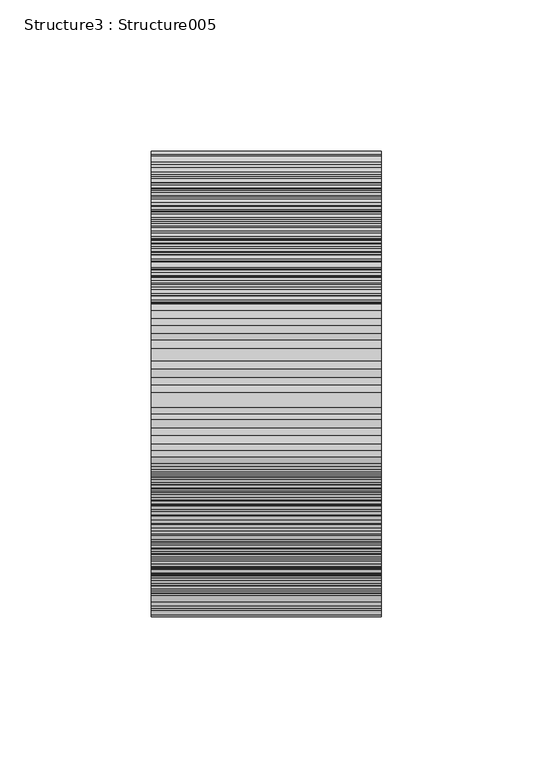
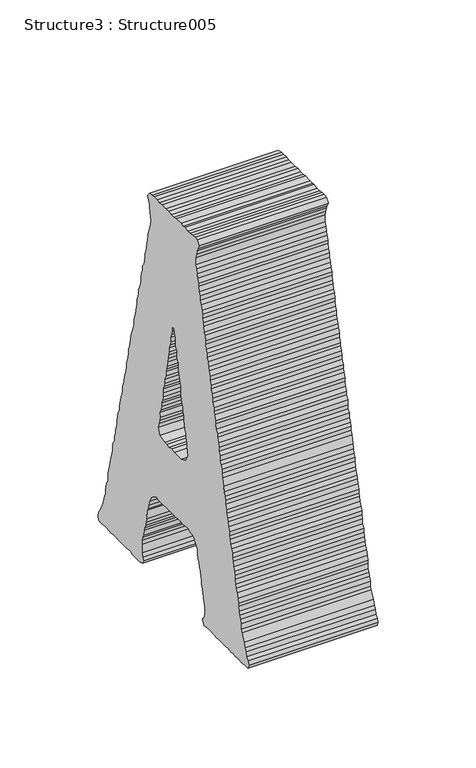
"""IFC4 building model written with IfcOpenShell, lengths in millimetres: proxy geometry, Structure3 : Structure005."""

from ifc_helpers import new_model, si_unit, frame, origin, place, context, project, spatial, polyline, outline, extrude, source, transform, mapped, element, save


def structure3_structure005_c6ac8972(model_context):
    return source(origin(), model_context, "Body", "SweptSolid", [
        extrude(outline(polyline([(2.1653931, 0.0), (4.9551582, -1.2360363), (7.1205514, -1.5418684), (9.8959144, -1.8477005), (12.3790002, -2.7770574), (14.2258535, -3.0947501), (17.0249376, -4.0122465), (19.4987044, -4.0122465), (22.2740675, -4.9424506), (24.4394606, -5.5659754), (27.2292257, -6.1776396), (29.3937717, -6.8011644), (31.8616083, -7.1069966), (33.7101559, -8.0363535), (36.8159193, -8.3430328), (38.9813125, -8.3430328), (41.7583699, -8.9665576), (43.3112516, -9.8959145), (46.4093904, -10.5194393), (48.2664099, -11.1311035), (50.7384823, -11.7546283), (53.207166, -11.7546283), (55.371712, -12.3671398), (58.1614771, -13.2964967), (60.6428686, -14.2258536), (63.419926, -14.2258536), (65.2676265, -15.1552105), (68.3750842, -15.7668748), (70.2219375, -15.7668748), (72.7041762, -16.6970789), (75.1770958, -17.0147715), (77.9524588, -17.6264358), (80.1322541, -18.5557927), (84.4621932, -18.5557927), (86.9291825, -17.9322679), (89.4029494, -17.3206037), (91.2591217, -16.3912467), (93.7311941, -15.1552105), (96.2142799, -17.3206037), (96.5226536, -19.4851496), (96.5226536, -21.6505428), (95.9109893, -24.4394607), (95.9109893, -26.9098388), (96.5226536, -29.6868962), (96.2142799, -31.54561), (96.5226536, -33.7110032), (96.5226536, -38.6644671), (95.9109893, -41.1356924), (95.9109893, -43.617931), (96.5226536, -46.3949884), (96.2142799, -49.1839063), (96.2142799, -53.1961528), (95.9109893, -55.9850707), (96.5226536, -58.1496167), (96.5226536, -60.9385346), (96.2142799, -63.1030806), (95.9109893, -65.8919985), (93.4245148, -67.739699), (91.2591217, -66.5036628), (89.0945757, -65.8919985), (87.2375562, -65.5743058), (84.4621932, -64.9626416), (79.8094783, -64.0332847), (77.6457795, -64.6449489), (74.8687221, -65.2684737), (69.9135639, -67.1271876), (68.3750842, -67.1271876), (65.5853191, -67.739699), (63.1166354, -68.3632238), (60.3268703, -68.6690559), (57.8437845, -69.2925807), (55.371712, -70.5277697), (53.5155397, -70.5277697), (50.7384823, -70.8336019), (48.2664099, -71.4579738), (46.4093904, -72.6931629), (43.6196253, -72.6931629), (41.1467056, -73.6225198), (38.9813125, -74.2460446), (36.5134759, -74.2460446), (33.7101559, -74.8577089), (31.2507912, -75.787913), (29.085398, -76.7172699), (27.2292257, -77.023102), (24.4394606, -77.3289341), (22.2740675, -78.258291), (19.4987044, -78.258291), (17.0249376, -79.1884951), (14.8510727, -79.4943273), (12.0748624, -80.1178521), (7.7322156, -81.6588732), (4.9551582, -81.6588732), (2.7906123, -82.282398), (0.3176926, -82.8949095), (-2.4720725, -84.141959), (-4.3282448, -84.4477912), (-6.8020116, -85.0594554), (-9.283403, -85.3771481), (-12.0604605, -86.306505), (-13.9217158, -86.9190165), (-16.7063979, -86.9190165), (-19.4826081, -87.8483734), (-21.3438635, -88.166066), (-24.1344758, -89.0835624), (-26.5929933, -89.4012551), (-29.0752319, -89.7070872), (-30.9322514, -90.330612), (-33.4136429, -91.2489556), (-36.4982268, -91.5666482), (-38.9711464, -92.1783125), (-40.5240281, -93.1076694), (-43.3002383, -93.1076694), (-46.0908506, -93.7311942), (-48.2553966, -94.6495378), (-51.0409258, -95.2730625), (-52.9021812, -95.8965873), (-55.0531722, -96.5082516), (-57.5354109, -96.5082516), (-60.6327025, -97.7553012), (-63.1013862, -98.3669654), (-65.2794871, -98.6736447), (-67.7524067, -98.6736447), (-69.6094262, -99.2971695), (-72.6931629, -100.2265264), (-74.5501824, -100.5323586), (-77.032421, -101.4617155), (-79.8128671, -101.4617155), (-81.9782603, -102.6977517), (-84.1428062, -103.3212765), (-86.6106428, -103.3212765), (-89.386853, -103.9448013), (-92.1910202, -104.8622977), (-94.3420113, -105.4858225), (-96.2032666, -106.1093473), (-98.9887958, -106.404166), (-101.4617155, -107.3453835), (-104.2514806, -107.9570477), (-106.7193172, -107.9570477), (-108.8982652, -108.2628799), (-111.0492563, -109.5099294), (-113.8390214, -110.1215937), (-116.311941, -110.7459657), (-118.476487, -110.7459657), (-120.6503519, -111.6753226), (-125.8994818, -113.2163438), (-128.0784298, -114.1457007), (-129.9261303, -115.0759048), (-132.7116595, -116.9346186), (-134.2560694, -117.5462829), (-137.0314325, -118.476487), (-139.2061446, -117.8639755), (-139.5136711, -114.7582121), (-139.2061446, -112.9105116), (-138.8884519, -110.1215937), (-139.5136711, -107.6512156), (-139.5136711, -104.8622977), (-138.8884519, -102.3910724), (-138.8884519, -100.2265264), (-139.2061446, -97.7553012), (-139.2061446, -95.5907552), (-139.5136711, -92.4841446), (-139.5136711, -90.330612), (-139.2061446, -87.8483734), (-138.8884519, -85.0594554), (-139.5136711, -82.8949095), (-139.5136711, -75.787913), (-138.8884519, -72.998995), (-136.7374609, -71.763806), (-134.8762055, -72.6931629), (-132.4083689, -73.3048272), (-127.1363652, -73.3048272), (-124.6634456, -73.3048272), (-122.4988996, -72.6931629), (-120.6503519, -71.763806), (-117.5437413, -71.4579738), (-115.3791954, -70.8336019), (-113.2138022, -69.904245), (-111.0492563, -69.2925807), (-108.5805725, -68.6690559), (-103.0145972, -68.0573916), (-101.4617155, -67.4338669), (-98.9887958, -66.5036628), (-95.8957401, -65.8919985), (-92.8018373, -64.3391168), (-90.9405819, -62.1737237), (-89.0928814, -58.7731415), (-89.7045457, -56.3027634), (-89.7045457, -51.3484523), (-89.386853, -48.2545494), (-89.386853, -41.7592171), (-89.7045457, -38.9702992), (-89.0928814, -36.8057533), (-89.386853, -34.334528), (-89.7045457, -31.8633027), (-89.386853, -29.6868962), (-89.0928814, -26.6040067), (-89.7045457, -24.7452928), (-90.6372913, -21.0388785), (-92.4943108, -19.167457), (-95.8957401, -16.6970789), (-98.6719504, -16.6970789), (-101.4617155, -16.0845674), (-103.0145972, -15.1552105), (-106.0991811, -14.8493784), (-107.9697554, -13.6023288), (-110.7459657, -12.9906646), (-112.6029851, -12.6848324), (-115.0759048, -12.6848324), (-117.5437413, -11.4369357), (-120.0302159, -11.1311035), (-122.4988996, -10.8252714), (-124.6634456, -9.8959145), (-127.7607372, -8.9665576), (-131.7831498, -9.2723897), (-134.8762055, -10.2017466), (-136.4206154, -11.7546283), (-139.5136711, -9.8959145), (-139.2061446, -7.1069966), (-138.8884519, -4.6366185), (-138.8884519, 0.3176926), (-139.2061446, 2.7880707), (-139.2061446, 5.259296), (-138.8884519, 7.4246891), (-139.2061446, 9.5892351), (-139.2061446, 12.6839852), (-138.8884519, 14.542699), (-139.2061446, 17.6374491), (-138.8884519, 19.4970101), (-139.5136711, 21.9673882), (-138.8884519, 24.7563061), (-139.5136711, 27.5333635), (-139.2061446, 29.6979095), (-138.8884519, 32.1809953), (-138.8884519, 34.6513734), (-136.4206154, 35.5815775), (-134.2560694, 34.9580527), (-132.7116595, 33.4161843), (-129.9261303, 32.7926595), (-128.0784298, 31.8633026), (-125.2742626, 30.6272664), (-120.6503519, 28.4627204), (-118.7797776, 27.8510562), (-115.7002768, 27.5333635), (-113.2138022, 26.9208521), (-111.0492563, 26.2973273), (-109.2015558, 25.3679704), (-106.0991811, 25.0621382), (-104.2514806, 25.0621382), (-101.4617155, 24.4386134), (-98.6719504, 23.5211171), (-96.5201121, 22.5790524), (-94.3420113, 21.9673882), (-91.565801, 21.661556), (-89.0928814, 21.3438634), (-86.9190164, 21.0380313), (-84.7629423, 19.8028422), (-81.6563317, 19.4970101), (-79.5053406, 19.1793174), (-77.032421, 18.8726381), (-74.858556, 17.9432812), (-72.3856364, 17.0139243), (-69.6094262, 16.40226), (-68.0556973, 15.7787352), (-65.5827776, 15.7787352), (-62.7980956, 14.8485311), (-60.0074833, 14.542699), (-58.151311, 13.9310347), (-55.6783914, 12.9898173), (-53.5223172, 12.6839852), (-50.7232331, 11.7664888), (-48.2553966, 11.7664888), (-46.0908506, 11.1421168), (-43.617931, 10.5304525), (-40.8273187, 9.9069278), (-36.1949362, 8.6598782), (-33.7220165, 8.0482139), (-31.2397779, 8.0482139), (-29.0752319, 7.1180098), (-26.910686, 6.1886529), (-23.8125472, 6.1886529), (-21.9690826, 4.9534639), (-19.4826081, 4.9534639), (-16.7063979, 4.6476317), (-14.2250064, 3.4115955), (-12.0604605, 3.4115955), (-9.9094694, 2.1764065), (-6.8020116, 1.8587138), (-4.6366185, 1.8587138), (-1.8612554, 0.6235247), (0.0, 0.0), (2.1653931, 0.0)]), holes=[polyline([(-49.7947234, -33.0993389), (-49.7947234, -40.2063354), (-49.5007518, -42.9944062), (-50.1124161, -45.7833241), (-49.5007518, -47.9487173), (-49.7947234, -50.1132632), (-48.2553966, -54.7490345), (-44.2423029, -56.3027634), (-41.1450113, -55.6792386), (-38.9711464, -55.0548666), (-36.8150722, -54.4432023), (-33.7220165, -54.7490345), (-31.5430685, -53.5138454), (-29.0752319, -53.1961528), (-26.910686, -52.8903206), (-24.7452928, -51.9728243), (-22.2639014, -51.6551316), (-19.7909818, -51.6551316), (-17.0147715, -51.3484523), (-15.1535162, -50.4190954), (-12.6848324, -49.7955706), (-10.203441, -49.7955706), (-7.4221477, -48.5603815), (-4.6366185, -48.5603815), (-2.4720725, -47.6310246), (-0.6099699, -47.3243453), (2.4737668, -47.0185132), (4.9551582, -46.3949884), (7.423842, -45.7833241), (9.5892351, -45.4656315), (12.0748624, -45.4656315), (14.5435462, -44.2304424), (16.7089393, -43.9246103), (19.4987044, -43.9246103), (21.9563748, -42.9944062), (24.1353229, -42.3827419), (26.300716, -42.3827419), (26.6040066, -41.4415245), (24.1353229, -40.8298602), (21.6496955, -39.9005033), (19.1810118, -39.593824), (16.4048016, -39.593824), (14.5435462, -38.358635), (11.7537811, -38.0409423), (9.8959144, -38.0409423), (7.423842, -36.8057533), (4.3307863, -36.4999211), (2.1653931, -36.194089), (0.0, -35.569717), (-2.4720725, -35.2638849), (-5.2567545, -34.334528), (-10.203441, -34.0286958), (-12.6848324, -33.4051711), (-15.1535162, -33.0993389), (-16.7063979, -32.169982), (-19.4826081, -32.169982), (-21.9690826, -30.9339458), (-24.4377663, -30.9339458), (-26.5929933, -30.310421), (-29.3920774, -30.0045889), (-31.2397779, -29.0752319), (-34.0159881, -29.0752319), (-36.8150722, -28.145875), (-38.6627727, -28.145875), (-41.1450113, -27.5215031), (-44.2423029, -26.9098388), (-47.9470229, -28.7693998), (-49.7947234, -33.0993389)])]), frame((-35624.0862846, 276259.8724527, 4122.0266343), z_axis=(1.0, 0.0, 1.354250045437766e-12), x_axis=(-1.354250045437766e-12, 0.0, 1.0)), (0.0, 0.0, 1.0), 76.2),
    ])


if __name__ == "__main__":
    model = new_model("IFC4")
    model_context = context("Model", 3, world=origin())
    ifc_project = project(units=[si_unit("LENGTHUNIT", "METRE", prefix="MILLI")], contexts=[model_context])
    site = spatial("IfcSite", under=ifc_project)
    building = spatial("IfcBuilding", under=site)
    placement = place(None, origin())
    structure3_structure005_shape = structure3_structure005_c6ac8972(model_context)
    element("IfcBuildingElementProxy", 1, Name="Structure3 : Structure005", ObjectType="Structure3 : Structure005", at=placement, inside=building, context=model_context, shape_type="MappedRepresentation", body=[
        mapped(structure3_structure005_shape, transform((0.0, 0.0, 0.0), x_axis=(1.0, 0.0, 0.0), y_axis=(0.0, 1.0, 0.0), z_axis=(0.0, 0.0, 1.0))),
    ])
    save(model, "model.ifc")

# Revit data of these elements
# Type "Structure3 : Structure005"
#   NameOverride = "Structure005"
# Element 1 (IfcBuildingElementProxy, "Structure3 : Structure005")
#   Materials on its faces: "BRUSHED ALUMINUM LETTERING"
# Materials
#   "BRUSHED ALUMINUM LETTERING": class "Unassigned", colour RGB 169 181 186, transparency 0, Cost = 0
